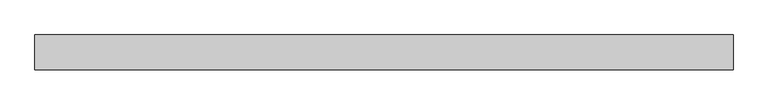
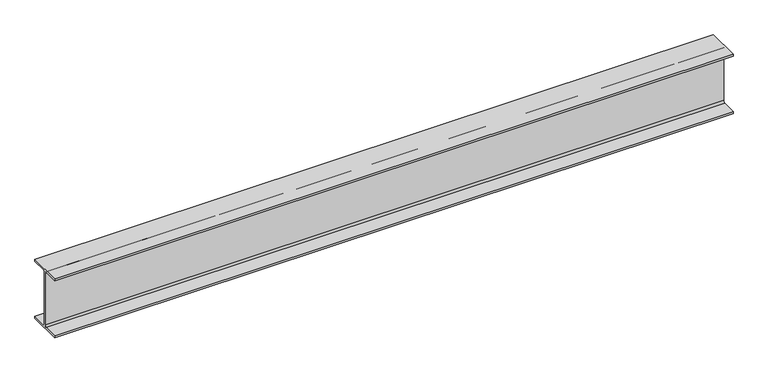
"""IFC4 building model written with IfcOpenShell, lengths in millimetres: beam geometry, Old_Steel Beam_H-KSD3502 : H_SB_ASB_H-200×200x8x12."""

import ifcopenshell
import ifcopenshell.guid

model = None  # the IFC model being written
_history = None  # IfcOwnerHistory: only IFC2X3 demands one
_inside = {}  # id of a spatial element -> (the spatial element, [elements in it])
_under = {}  # id of a project, library or spatial element -> (it, [spatial elements below it])
_declared = {}  # id of a project -> (the project, [libraries it declares])
_typed = {}  # id of a type object -> (the type object, [elements of that type])
_made_of = {}  # id of a material, layer set ... -> (it, [elements and type objects made of it])


def new_model(schema):
    """Start an empty IFC model of exactly this schema.

    Asked for "IFC4X3", IfcOpenShell would pick the latest addendum, in which some entities
    have other attributes; the version numbers below select the first issue.
    IFC2X3 requires an IfcOwnerHistory on every rooted entity: one is made here for all.
    """
    global model, _history
    if schema == "IFC4X3":
        model = ifcopenshell.file(schema_version=(4, 3, 0, 0))
    else:
        model = ifcopenshell.file(schema=schema)
    _inside.clear()
    _under.clear()
    _declared.clear()
    _typed.clear()
    _made_of.clear()
    _history = None
    if model.schema == "IFC2X3":
        org = make("IfcOrganization", Name="unknown")
        user = make(
            "IfcPersonAndOrganization",
            ThePerson=make("IfcPerson", FamilyName="unknown"),
            TheOrganization=org,
        )
        app = make(
            "IfcApplication",
            ApplicationDeveloper=org,
            Version="unknown",
            ApplicationFullName="unknown",
            ApplicationIdentifier="unknown",
        )
        _history = make(
            "IfcOwnerHistory",
            OwningUser=user,
            OwningApplication=app,
            ChangeAction="ADDED",
            CreationDate=0,
        )
    return model


def make(cls, **values):
    """One entity of the class cls with the attributes given. An attribute that is None is left unset."""
    return model.create_entity(
        cls, **{name: value for name, value in values.items() if value is not None}
    )


def rooted(cls, **values):
    """An entity with a GlobalId (a new one), such as an element, a storey or a relation."""
    return make(cls, GlobalId=ifcopenshell.guid.new(), OwnerHistory=_history, **values)


def si_unit(unit_type, name, prefix=None):
    """IfcSIUnit, for example si_unit("LENGTHUNIT", "METRE", prefix="MILLI")."""
    return make("IfcSIUnit", UnitType=unit_type, Prefix=prefix, Name=name)


def assignment(units):
    """IfcUnitAssignment: the units of a project."""
    return None if units is None else make("IfcUnitAssignment", Units=units)


def point(xyz):
    """IfcCartesianPoint."""
    return None if xyz is None else make("IfcCartesianPoint", Coordinates=xyz)


def direction(xyz):
    """IfcDirection."""
    return None if xyz is None else make("IfcDirection", DirectionRatios=xyz)


def frame(location, z_axis=None, x_axis=None):
    """IfcAxis2Placement3D, a coordinate frame: its origin and axes. An axis left out is left unset."""
    return make(
        "IfcAxis2Placement3D",
        Location=point(location),
        Axis=direction(z_axis),
        RefDirection=direction(x_axis),
    )


def frame_2d(location, x_axis=None):
    """IfcAxis2Placement2D, a coordinate frame in the plane: its origin and x axis."""
    return make(
        "IfcAxis2Placement2D", Location=point(location), RefDirection=direction(x_axis)
    )


def origin():
    """The frame at (0, 0, 0) with its axes left unset."""
    return frame((0.0, 0.0, 0.0))


def place(relative_to, where):
    """IfcLocalPlacement: puts the frame where relative to a parent placement (None: the world)."""
    return make(
        "IfcLocalPlacement", PlacementRelTo=relative_to, RelativePlacement=where
    )


def context(
    kind, dimensions, precision=None, world=None, true_north=None, identifier=None
):
    """IfcGeometricRepresentationContext, for example the 3D "Model" context."""
    return make(
        "IfcGeometricRepresentationContext",
        ContextIdentifier=identifier,
        ContextType=kind,
        CoordinateSpaceDimension=dimensions,
        Precision=precision,
        WorldCoordinateSystem=world,
        TrueNorth=true_north,
    )


def project(units=None, contexts=None):
    """IfcProject with its units and contexts."""
    return rooted(
        "IfcProject",
        Name="project",
        RepresentationContexts=contexts,
        UnitsInContext=assignment(units),
    )


def spatial(cls, under=None, at=None, **own):
    """A site, building, storey or space (cls), placed at a placement, below another one or the project."""
    s = rooted(cls, ObjectPlacement=at, **own)
    if under is not None:
        _under.setdefault(under.id(), (under, []))[1].append(s)
    return s


def polyline(points):
    """IfcPolyline through the points."""
    return make("IfcPolyline", Points=[point(p) for p in points])


def circle_curve(where, radius):
    """IfcCircle in the frame where."""
    return make("IfcCircle", Position=where, Radius=radius)


def trimmed(basis, trim1, trim2, sense, master):
    """IfcTrimmedCurve: the piece of a basis curve between two trims."""
    return make(
        "IfcTrimmedCurve",
        BasisCurve=basis,
        Trim1=trim1,
        Trim2=trim2,
        SenseAgreement=sense,
        MasterRepresentation=master,
    )


def segment(curve, same_sense, transition):
    """IfcCompositeCurveSegment."""
    return make(
        "IfcCompositeCurveSegment",
        Transition=transition,
        SameSense=same_sense,
        ParentCurve=curve,
    )


def composite_curve(segments, self_intersect=None):
    """IfcCompositeCurve: segments joined end to end."""
    return make("IfcCompositeCurve", Segments=segments, SelfIntersect=self_intersect)


def outline(outer, holes=None, kind="AREA"):
    """IfcArbitraryClosedProfileDef: a profile drawn as a closed curve; with holes, ...WithVoids."""
    if holes is None:
        return make("IfcArbitraryClosedProfileDef", ProfileType=kind, OuterCurve=outer)
    return make(
        "IfcArbitraryProfileDefWithVoids",
        ProfileType=kind,
        OuterCurve=outer,
        InnerCurves=holes,
    )


def extrude(swept, where, along, depth):
    """IfcExtrudedAreaSolid: the profile swept, set in the frame where, extruded along a direction by depth."""
    return make(
        "IfcExtrudedAreaSolid",
        SweptArea=swept,
        Position=where,
        ExtrudedDirection=direction(along),
        Depth=depth,
    )


def shape(context_of_items, identifier, shape_type, items):
    """IfcShapeRepresentation: the items that make up one representation, for example the "Body"."""
    return make(
        "IfcShapeRepresentation",
        ContextOfItems=context_of_items,
        RepresentationIdentifier=identifier,
        RepresentationType=shape_type,
        Items=items,
    )


def source(mapping_origin, context_of_items, identifier, shape_type, items):
    """IfcRepresentationMap: a shape defined once, which mapped items show again and again."""
    return make(
        "IfcRepresentationMap",
        MappingOrigin=mapping_origin,
        MappedRepresentation=shape(context_of_items, identifier, shape_type, items),
    )


def transform(
    local_origin,
    x_axis=None,
    y_axis=None,
    z_axis=None,
    scale=None,
    scale2=None,
    scale3=None,
    uniform=True,
):
    """IfcCartesianTransformationOperator3D, or its non-uniform kind. x_axis, y_axis, z_axis: its Axis1, 2, 3."""
    if uniform:
        return make(
            "IfcCartesianTransformationOperator3D",
            Axis1=direction(x_axis),
            Axis2=direction(y_axis),
            LocalOrigin=point(local_origin),
            Scale=scale,
            Axis3=direction(z_axis),
        )
    return make(
        "IfcCartesianTransformationOperator3DnonUniform",
        Axis1=direction(x_axis),
        Axis2=direction(y_axis),
        LocalOrigin=point(local_origin),
        Scale=scale,
        Axis3=direction(z_axis),
        Scale2=scale2,
        Scale3=scale3,
    )


def mapped(mapping_source, mapping_target):
    """IfcMappedItem: shows the shape of a source again, moved by a transform."""
    return make(
        "IfcMappedItem", MappingSource=mapping_source, MappingTarget=mapping_target
    )


def made_of(thing, what):
    """Note that an element or type object is made of a material, layer set ...; save() writes the relation."""
    if what is not None:
        _made_of.setdefault(what.id(), (what, []))[1].append(thing)
    return thing


def element(
    cls,
    number,
    at=None,
    inside=None,
    cuts=None,
    type_object=None,
    material=None,
    context=None,
    identifier="Body",
    shape_type=None,
    held_by="IfcProductDefinitionShape",
    body=None,
    shapes=None,
    **own,
):
    """One element of the class cls, such as IfcWall. Its Tag is "e" and its number.

    at: its placement. inside: the storey or other place that contains it. cuts: it is an
    opening in that element (IfcRelVoidsElement). A single representation is given by context,
    identifier, shape_type and body (its items); several are given by shapes. held_by: the class
    of the entity that holds the representations. save() writes the other relations.
    """
    e = rooted(cls, Tag="e%d" % number, ObjectPlacement=at, **own)
    if body is not None:
        shapes = [shape(context, identifier, shape_type, body)]
    if shapes is not None:
        e.Representation = make(held_by, Representations=shapes)
    if inside is not None:
        _inside.setdefault(inside.id(), (inside, []))[1].append(e)
    if cuts is not None:
        rooted(
            "IfcRelVoidsElement", RelatingBuildingElement=cuts, RelatedOpeningElement=e
        )
    if type_object is not None:
        _typed.setdefault(type_object.id(), (type_object, []))[1].append(e)
    return made_of(e, material)


def aggregate(whole, parts):
    """IfcRelAggregates: a whole, such as a stair, and the parts it consists of."""
    return rooted("IfcRelAggregates", RelatingObject=whole, RelatedObjects=parts)


def save(model, path):
    """Write the relations noted so far, then the file.

    IfcRelAggregates (storeys below a building ...), IfcRelContainedInSpatialStructure (elements
    in a storey), IfcRelDefinesByType, IfcRelAssociatesMaterial and IfcRelDeclares: one each for
    every whole, place, type object, material and project.
    """
    for whole, parts in _under.values():
        aggregate(whole, parts)
    for where, things in _inside.values():
        rooted(
            "IfcRelContainedInSpatialStructure",
            RelatedElements=things,
            RelatingStructure=where,
        )
    for kind, things in _typed.values():
        rooted("IfcRelDefinesByType", RelatedObjects=things, RelatingType=kind)
    for what, things in _made_of.values():
        rooted("IfcRelAssociatesMaterial", RelatedObjects=things, RelatingMaterial=what)
    for by, libraries in _declared.values():
        rooted("IfcRelDeclares", RelatingContext=by, RelatedDefinitions=libraries)
    model.write(path)


def beam_ca562099(model_context):
    return source(origin(), model_context, "Body", "SweptSolid", [
        extrude(outline(composite_curve([segment(polyline([(82.5, -141.5), (82.5, -151.7), (-82.5, -151.7), (-82.5, -141.5), (-11.9, -141.5)]), True, "CONTINUOUS"), segment(trimmed(circle_curve(frame_2d((-11.9, -132.6)), 8.9), [point((-11.9, -141.5))], [point((-3.0, -132.6))], True, "CARTESIAN"), True, "CONTINUOUS"), segment(polyline([(-3.0, -132.6), (-3.0, 132.6)]), True, "CONTINUOUS"), segment(trimmed(circle_curve(frame_2d((-11.9, 132.6)), 8.9), [point((-3.0, 132.6))], [point((-11.9, 141.5))], True, "CARTESIAN"), True, "CONTINUOUS"), segment(polyline([(-11.9, 141.5), (-82.5, 141.5), (-82.5, 151.7), (82.5, 151.7), (82.5, 141.5), (11.9, 141.5)]), True, "CONTINUOUS"), segment(trimmed(circle_curve(frame_2d((11.9, 132.6)), 8.9), [point((11.9, 141.5))], [point((3.0, 132.6))], True, "CARTESIAN"), True, "CONTINUOUS"), segment(polyline([(3.0, 132.6), (3.0, -132.6)]), True, "CONTINUOUS"), segment(trimmed(circle_curve(frame_2d((11.9, -132.6)), 8.9), [point((3.0, -132.6))], [point((11.9, -141.5))], True, "CARTESIAN"), True, "CONTINUOUS"), segment(polyline([(11.9, -141.5), (82.5, -141.5)]), True, "CONTINUOUS")], self_intersect=False)), frame((-1452.9542052, 0.0, 0.0), z_axis=(1.0, 0.0, 0.0), x_axis=(0.0, 1.0, 0.0)), (0.0, 0.0, 1.0), 3291.2393621),
    ])


if __name__ == "__main__":
    model = new_model("IFC4")
    model_context = context("Model", 3, world=origin())
    ifc_project = project(units=[si_unit("LENGTHUNIT", "METRE", prefix="MILLI")], contexts=[model_context])
    site = spatial("IfcSite", under=ifc_project)
    building = spatial("IfcBuilding", under=site)
    placement = place(None, origin())
    beam_shape = beam_ca562099(model_context)
    element("IfcBeam", 1, ObjectType="Old_Steel Beam_H-KSD3502 : H_SB_ASB_H-200×200x8x12", at=placement, inside=building, context=model_context, shape_type="MappedRepresentation", body=[
        mapped(beam_shape, transform((0.0, 0.0, 0.0), x_axis=(1.0, 0.0, 0.0), y_axis=(0.0, 1.0, 0.0), z_axis=(0.0, 0.0, 1.0))),
    ])
    save(model, "model.ifc")

# Revit data of these elements
# Type "Old_Steel Beam_H-KSD3502 : H_SB_ASB_H-200×200x8x12"
#   Width = 20.0 cm
#   Web Thickness = 0.8 cm
#   Web Fillet = 1.3 cm
#   Warping Constant = 141376.0 cm⁶
#   Torsional Moment of Inertia = 26.2485 cm⁴
#   Torsional Modulus = 1.0 cm³
#   Section Area = 63.53 cm²
#   Plastic Modulus weak axis = 244.0 cm³
#   Plastic Modulus strong axis = 525.0 cm³
#   Perimeter = 1.16 m²/m
#   Nominal Weight = 49.90 kgf/m
#   Moment of Inertia weak axis = 1600.00 cm⁴
#   Moment of Inertia strong axis = 4720.00 cm⁴
#   Height = 20.0 cm
#   Flange Thickness = 1.2 cm
#   Elastic Modulus weak axis = 160.0 cm³
#   Elastic Modulus strong axis = 472.0 cm³
#   Centroid Vertical = 10.0 cm
#   Centroid Horizontal = 10.0 cm
#   Length [instance default] = 1.5240 m
#   Structural Material [instance default] = Steel, 45-345
#   Assembly Code = ""
# Element 1 (IfcBeam, "Old_Steel Beam_H-KSD3502 : H_SB_ASB_H-200×200x8x12")
#   Structural Material = none
# Materials
#   "Steel, 45-345": class "Metal", colour RGB 189 187 185, transparency 0, Description = "Steel 345 MPa", Cost = 0
